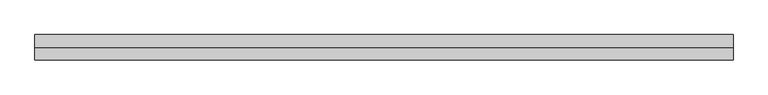
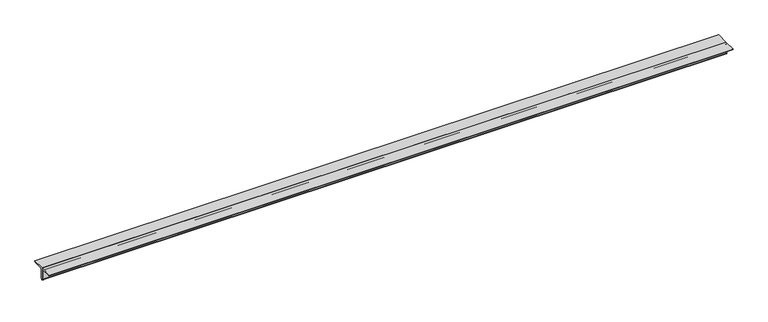
"""IFC4 building model written with IfcOpenShell, lengths in millimetres: beam geometry, 0123_Steel Framing_2Ls-KSD3502 : H_SB_AR_S04_2Ls-130x130x12_VBR2."""

from ifc_helpers import new_model, si_unit, point, frame, frame_2d, origin, place, context, project, spatial, polyline, circle_curve, trimmed, segment, composite_curve, outline, extrude, source, transform, mapped, element, save


def beam_9327e08a(model_context):
    return source(origin(), model_context, "Body", "SweptSolid", [
        extrude(outline(composite_curve([segment(polyline([(0.0, 36.4), (130.0, 36.4)]), True, "CONTINUOUS"), segment(trimmed(circle_curve(frame_2d((118.0, 36.4)), 12.0), [point((130.0, 36.4))], [point((118.0, 24.4))], False, "CARTESIAN"), True, "CONTINUOUS"), segment(polyline([(118.0, 24.4), (24.0, 24.4)]), True, "CONTINUOUS"), segment(trimmed(circle_curve(frame_2d((24.0, 12.4)), 12.0), [point((24.0, 24.4))], [point((12.0, 12.4))], True, "CARTESIAN"), True, "CONTINUOUS"), segment(polyline([(12.0, 12.4), (12.0, -81.6)]), True, "CONTINUOUS"), segment(trimmed(circle_curve(frame_2d((0.0, -81.6)), 12.0), [point((12.0, -81.6))], [point((0.0, -93.6))], False, "CARTESIAN"), True, "CONTINUOUS"), segment(polyline([(0.0, -93.6), (0.0, 36.4)]), True, "CONTINUOUS")], self_intersect=False)), frame((-3534.7173983, 0.0, 0.0), z_axis=(1.0, 0.0, 0.0), x_axis=(0.0, 1.0, 0.0)), (0.0, 0.0, 1.0), 7187.6786398),
        extrude(outline(composite_curve([segment(polyline([(0.0, 36.4), (0.0, -93.6)]), True, "CONTINUOUS"), segment(trimmed(circle_curve(frame_2d((0.0, -81.6)), 12.0), [point((0.0, -93.6))], [point((-12.0, -81.6))], False, "CARTESIAN"), True, "CONTINUOUS"), segment(polyline([(-12.0, -81.6), (-12.0, 12.4)]), True, "CONTINUOUS"), segment(trimmed(circle_curve(frame_2d((-24.0, 12.4)), 12.0), [point((-12.0, 12.4))], [point((-24.0, 24.4))], True, "CARTESIAN"), True, "CONTINUOUS"), segment(polyline([(-24.0, 24.4), (-118.0, 24.4)]), True, "CONTINUOUS"), segment(trimmed(circle_curve(frame_2d((-118.0, 36.4)), 12.0), [point((-118.0, 24.4))], [point((-130.0, 36.4))], False, "CARTESIAN"), True, "CONTINUOUS"), segment(polyline([(-130.0, 36.4), (0.0, 36.4)]), True, "CONTINUOUS")], self_intersect=False)), frame((-3534.7173983, 0.0, 0.0), z_axis=(1.0, 0.0, 0.0), x_axis=(0.0, 1.0, 0.0)), (0.0, 0.0, 1.0), 7187.6786398),
    ])


if __name__ == "__main__":
    model = new_model("IFC4")
    model_context = context("Model", 3, world=origin())
    ifc_project = project(units=[si_unit("LENGTHUNIT", "METRE", prefix="MILLI")], contexts=[model_context])
    site = spatial("IfcSite", under=ifc_project)
    building = spatial("IfcBuilding", under=site)
    placement = place(None, origin())
    beam_shape = beam_9327e08a(model_context)
    element("IfcBeam", 1, ObjectType="0123_Steel Framing_2Ls-KSD3502 : H_SB_AR_S04_2Ls-130x130x12_VBR2", at=placement, inside=building, context=model_context, shape_type="MappedRepresentation", body=[
        mapped(beam_shape, transform((0.0, 0.0, 0.0), x_axis=(1.0, 0.0, 0.0), y_axis=(0.0, 1.0, 0.0), z_axis=(0.0, 0.0, 1.0))),
    ])
    save(model, "model.ifc")

# Revit data of these elements
# Type "0123_Steel Framing_2Ls-KSD3502 : H_SB_AR_S04_2Ls-130x130x12_VBR2"
#   Type Mark = "VBR2"
#   Assembly Code = "B10"
#   Legs = "SLBB"
#   W = 8.97
#   Perimeter = 1.04 m²/m
#   Nominal Weight = 46.80 kgf/m
#   Length [instance default] = 1000 mm
#   Space = 0 mm
#   b = 130 mm
#   d = 130 mm
#   t = 12 mm
#   y = 36.4 mm
#   A = 0.005952 m²
#   Structural Material [instance default] = Steel ASTM A36
# Element 1 (IfcBeam, "0123_Steel Framing_2Ls-KSD3502 : H_SB_AR_S04_2Ls-130x130x12_VBR2")
#   Materials on its faces: "Steel ASTM A36"
# Materials
#   "Steel ASTM A36": class "Metal", colour RGB 199 199 199, transparency 0, Description = "Structural steel, ASTM A36 Grade B, mill finish", Cost = 0
